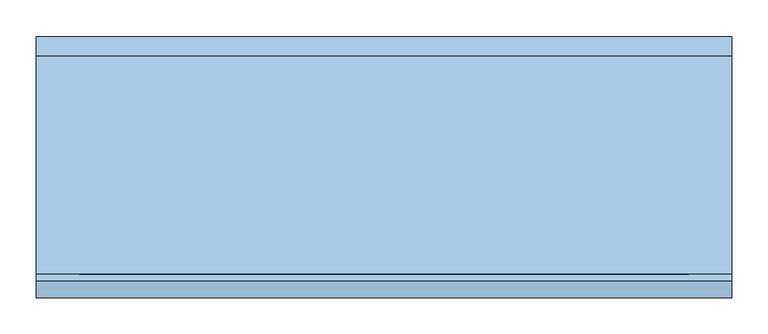
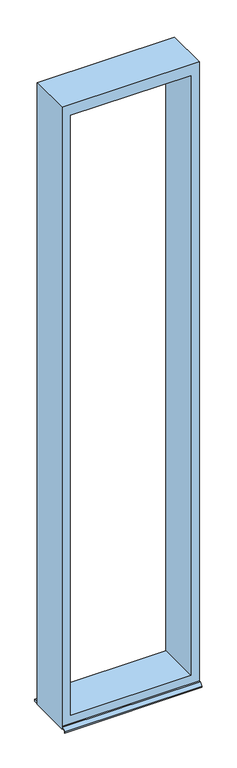
"""IFC4 building model written with IfcOpenShell, lengths in millimetres: window geometry, Fenster - Festverglasung : Feste Verglasung 4.58 x 0.96 2."""

from ifc_helpers import new_model, si_unit, frame, origin, place, context, project, spatial, polyline, outline, extrude, source, transform, mapped, element, save


def window_814c17b3(model_context):
    return source(origin(), model_context, "Body", "SweptSolid", [
        extrude(outline(polyline([(5580.0, 480.0), (5580.0, -480.0), (1000.0, -480.0), (1000.0, 480.0), (5580.0, 480.0)]), holes=[polyline([(5500.0, 420.0), (1080.0, 420.0), (1080.0, -420.0), (5500.0, -420.0), (5500.0, 420.0)])]), frame((0.0, -147.5214598, 0.0), z_axis=(0.0, 1.0, 0.0), x_axis=(0.0, 0.0, 1.0)), (0.0, 0.0, 1.0), 300.0),
        extrude(outline(polyline([(-480.0, 180.0), (480.0, 180.0), (480.0, 152.4785402), (-480.0, 152.4785402), (-480.0, 180.0)])), frame((0.0, 0.0, 1005.0), z_axis=(0.0, 0.0, 1.0), x_axis=(1.0, 0.0, 0.0)), (0.0, 0.0, 1.0), 15.0),
        extrude(outline(polyline([(-157.5436142, 1020.0), (-147.5214598, 1020.0), (-147.5214598, 1018.0), (-157.3455321, 1018.0), (-178.0, 998.3604634), (-178.0, 990.0), (-180.0, 990.0), (-180.0, 1000.0), (-157.5436142, 1020.0)])), frame((-480.0, 0.0, 0.0), z_axis=(1.0, 0.0, 0.0), x_axis=(0.0, 1.0, 0.0)), (0.0, 0.0, 1.0), 960.0),
    ])


if __name__ == "__main__":
    model = new_model("IFC4")
    model_context = context("Model", 3, world=origin())
    ifc_project = project(units=[si_unit("LENGTHUNIT", "METRE", prefix="MILLI")], contexts=[model_context])
    site = spatial("IfcSite", under=ifc_project)
    building = spatial("IfcBuilding", under=site)
    placement = place(None, origin())
    window_shape = window_814c17b3(model_context)
    element("IfcWindow", 1, ObjectType="Fenster - Festverglasung : Feste Verglasung 4.58 x 0.96 2", at=placement, inside=building, context=model_context, shape_type="MappedRepresentation", body=[
        mapped(window_shape, transform((0.0, 0.0, 0.0), x_axis=(1.0, 0.0, 0.0), y_axis=(0.0, 1.0, 0.0), z_axis=(0.0, 0.0, 1.0))),
    ])
    save(model, "model.ifc")

# Revit data of these elements
# Type "Fenster - Festverglasung : Feste Verglasung 4.58 x 0.96 2"
#   Type Mark = "70"
#   Operation = "SinglePanel"
#   Keynote = "16.05.01"
#   Visual Light Transmittance = 0.9
#   Solar Heat Gain Coefficient = 0.78
#   Rough Width = 0.960 m
#   Rough Height = 4.580 m
#   Heat Transfer Coefficient (U) = 3.6886 W/(m²·K)
#   Rahmentiefe = 0.300 m
#   Rahmenhöhe unten = 0.080 m
#   Höhe oberer  Rahmen = 0.080 m
#   Rahmenbreite = 0.060 m
#   Height = 4.580 m
#   Einbautiefe (von außen) [instance default] = 0.080 m
#   Width = 0.960 m
#   Wall Closure = 3
#   Bild [instance default] = none
#   Glas [instance default] = none
#   Innere Fensterbank [instance default] = none
#   Äußere Fensterbank [instance default] = none
#   Construction Type Id = ""
#   Analytic Construction = (empty or 0)
# Element 1 (IfcWindow, "Fenster - Festverglasung : Feste Verglasung 4.58 x 0.96 2")
#   Einbautiefe (von außen) = 0.002479 m
#   Materials on its faces: "Kunststoff - Weiß", "Holz - Birke"
# Materials
#   "Kunststoff - Weiß": class "Kunststoff", colour RGB 249 249 249, transparency 0, Cost = 0
#   "Holz - Birke": class "Holz", colour RGB 213 164 103, transparency 0, Cost = 0
